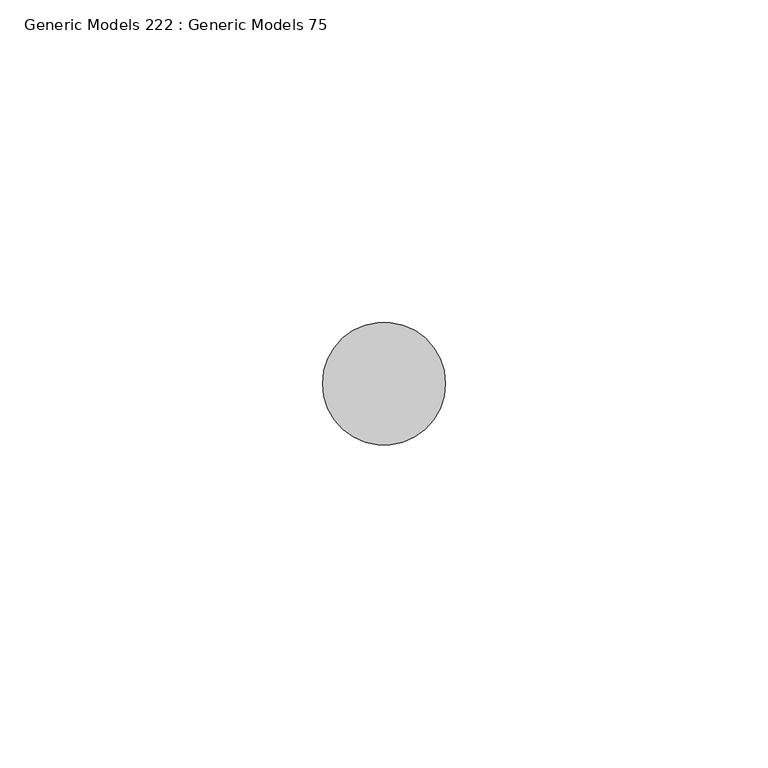
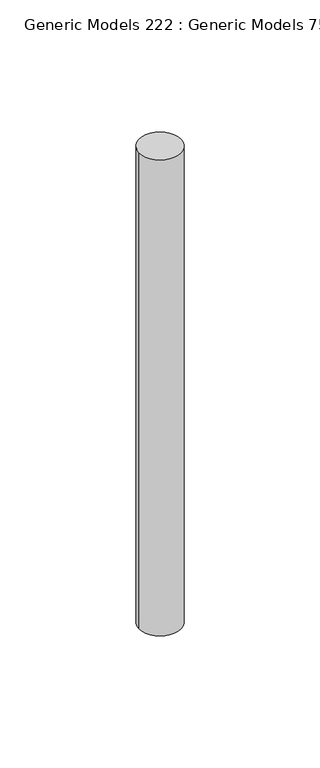
"""IFC4 building model written with IfcOpenShell, lengths in millimetres: proxy geometry, Generic Models 222 : Generic Models 75."""

from ifc_helpers import new_model, si_unit, point, frame, frame_2d, origin, place, context, project, spatial, circle_curve, trimmed, segment, composite_curve, outline, extrude, source, transform, mapped, element, save


def generic_models_222_generic_models_75_2b5840a4(model_context):
    return source(origin(), model_context, "Body", "SweptSolid", [
        extrude(outline(composite_curve([segment(trimmed(circle_curve(frame_2d((31975.4096032, 30896.6257369)), 9.525), [point((31965.8846032, 30896.6257369))], [point((31984.9346032, 30896.6257369))], False, "CARTESIAN"), True, "CONTINUOUS"), segment(trimmed(circle_curve(frame_2d((31975.4096032, 30896.6257369)), 9.525), [point((31984.9346032, 30896.6257369))], [point((31965.8846032, 30896.6257369))], False, "CARTESIAN"), True, "CONTINUOUS")], self_intersect=False)), frame((0.0, 0.0, 266211.05), z_axis=(0.0, 0.0, 1.0), x_axis=(1.0, 0.0, 0.0)), (0.0, 0.0, 1.0), 228.6),
    ])


if __name__ == "__main__":
    model = new_model("IFC4")
    model_context = context("Model", 3, world=origin())
    ifc_project = project(units=[si_unit("LENGTHUNIT", "METRE", prefix="MILLI")], contexts=[model_context])
    site = spatial("IfcSite", under=ifc_project)
    building = spatial("IfcBuilding", under=site)
    placement = place(None, origin())
    generic_models_222_generic_models_75_shape = generic_models_222_generic_models_75_2b5840a4(model_context)
    element("IfcBuildingElementProxy", 1, Name="Generic Models 222 : Generic Models 75", ObjectType="Generic Models 222 : Generic Models 75", at=placement, inside=building, context=model_context, shape_type="MappedRepresentation", body=[
        mapped(generic_models_222_generic_models_75_shape, transform((0.0, 0.0, 0.0), x_axis=(1.0, 0.0, 0.0), y_axis=(0.0, 1.0, 0.0), z_axis=(0.0, 0.0, 1.0))),
    ])
    save(model, "model.ifc")

# Revit data of these elements
# Element 1 (IfcBuildingElementProxy, "Generic Models 222 : Generic Models 75")
#   Materials on its faces: "5/8\" DIA. EPOXY ANCHOR BOLTS"
# Materials
#   "5/8\" DIA. EPOXY ANCHOR BOLTS": class "Metal", colour RGB 199 199 199, transparency 0, Description = "Carbon steel", Cost = 0
